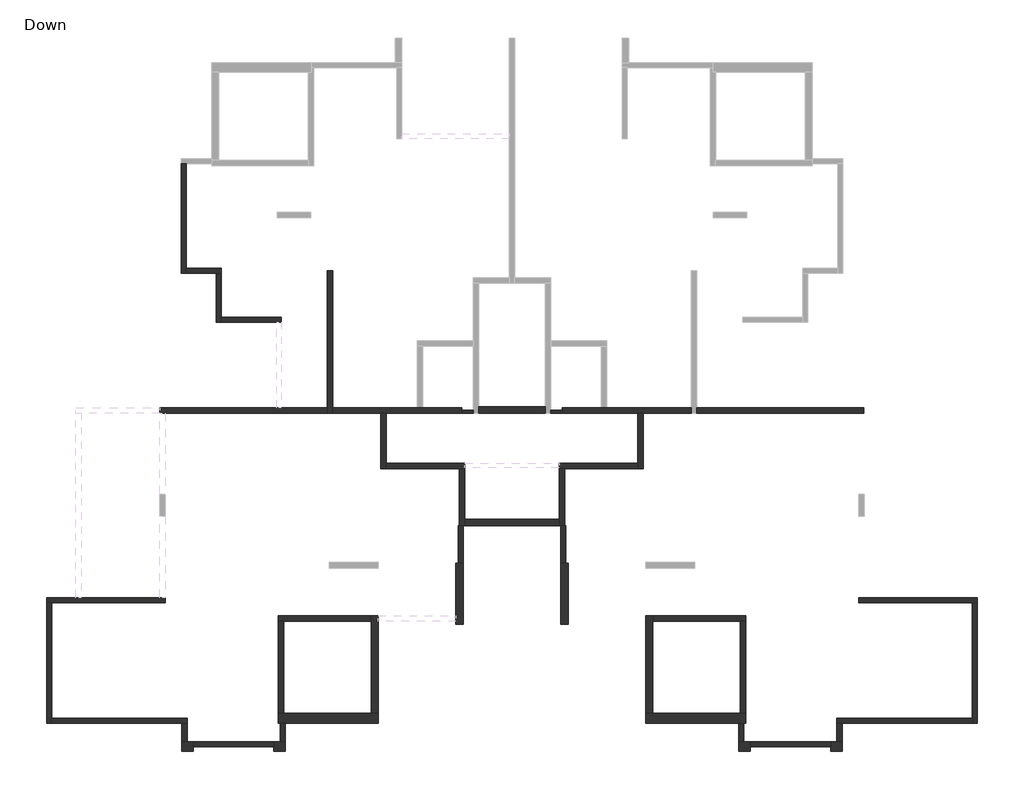
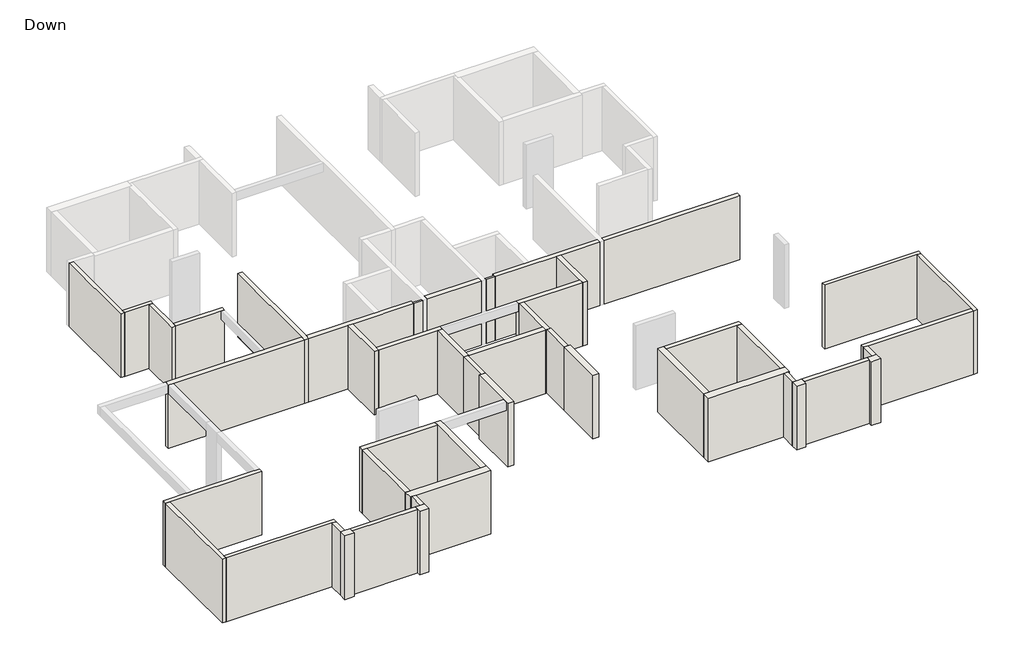
# One storey, part 1 of 2: 47 walls.
"""IFC4 building model written with IfcOpenShell, lengths in millimetres."""

import ifcopenshell
import ifcopenshell.guid

model = None  # the IFC model being written
_history = None  # IfcOwnerHistory: only IFC2X3 demands one
_inside = {}  # id of a spatial element -> (the spatial element, [elements in it])
_under = {}  # id of a project, library or spatial element -> (it, [spatial elements below it])
_declared = {}  # id of a project -> (the project, [libraries it declares])
_typed = {}  # id of a type object -> (the type object, [elements of that type])
_made_of = {}  # id of a material, layer set ... -> (it, [elements and type objects made of it])


def new_model(schema):
    """Start an empty IFC model of exactly this schema.

    Asked for "IFC4X3", IfcOpenShell would pick the latest addendum, in which some entities
    have other attributes; the version numbers below select the first issue.
    IFC2X3 requires an IfcOwnerHistory on every rooted entity: one is made here for all.
    """
    global model, _history
    if schema == "IFC4X3":
        model = ifcopenshell.file(schema_version=(4, 3, 0, 0))
    else:
        model = ifcopenshell.file(schema=schema)
    _inside.clear()
    _under.clear()
    _declared.clear()
    _typed.clear()
    _made_of.clear()
    _history = None
    if model.schema == "IFC2X3":
        org = make("IfcOrganization", Name="unknown")
        user = make(
            "IfcPersonAndOrganization",
            ThePerson=make("IfcPerson", FamilyName="unknown"),
            TheOrganization=org,
        )
        app = make(
            "IfcApplication",
            ApplicationDeveloper=org,
            Version="unknown",
            ApplicationFullName="unknown",
            ApplicationIdentifier="unknown",
        )
        _history = make(
            "IfcOwnerHistory",
            OwningUser=user,
            OwningApplication=app,
            ChangeAction="ADDED",
            CreationDate=0,
        )
    return model


def make(cls, **values):
    """One entity of the class cls with the attributes given. An attribute that is None is left unset."""
    return model.create_entity(
        cls, **{name: value for name, value in values.items() if value is not None}
    )


def rooted(cls, **values):
    """An entity with a GlobalId (a new one), such as an element, a storey or a relation."""
    return make(cls, GlobalId=ifcopenshell.guid.new(), OwnerHistory=_history, **values)


def si_unit(unit_type, name, prefix=None):
    """IfcSIUnit, for example si_unit("LENGTHUNIT", "METRE", prefix="MILLI")."""
    return make("IfcSIUnit", UnitType=unit_type, Prefix=prefix, Name=name)


def assignment(units):
    """IfcUnitAssignment: the units of a project."""
    return None if units is None else make("IfcUnitAssignment", Units=units)


def point(xyz):
    """IfcCartesianPoint."""
    return None if xyz is None else make("IfcCartesianPoint", Coordinates=xyz)


def direction(xyz):
    """IfcDirection."""
    return None if xyz is None else make("IfcDirection", DirectionRatios=xyz)


def frame(location, z_axis=None, x_axis=None):
    """IfcAxis2Placement3D, a coordinate frame: its origin and axes. An axis left out is left unset."""
    return make(
        "IfcAxis2Placement3D",
        Location=point(location),
        Axis=direction(z_axis),
        RefDirection=direction(x_axis),
    )


def origin():
    """The frame at (0, 0, 0) with its axes left unset."""
    return frame((0.0, 0.0, 0.0))


def origin_with_axes():
    """The frame at (0, 0, 0) with the z axis (0, 0, 1) and the x axis (1, 0, 0) written out."""
    return frame((0.0, 0.0, 0.0), z_axis=(0.0, 0.0, 1.0), x_axis=(1.0, 0.0, 0.0))


def place(relative_to, where):
    """IfcLocalPlacement: puts the frame where relative to a parent placement (None: the world)."""
    return make(
        "IfcLocalPlacement", PlacementRelTo=relative_to, RelativePlacement=where
    )


def context(
    kind, dimensions, precision=None, world=None, true_north=None, identifier=None
):
    """IfcGeometricRepresentationContext, for example the 3D "Model" context."""
    return make(
        "IfcGeometricRepresentationContext",
        ContextIdentifier=identifier,
        ContextType=kind,
        CoordinateSpaceDimension=dimensions,
        Precision=precision,
        WorldCoordinateSystem=world,
        TrueNorth=true_north,
    )


def project(units=None, contexts=None):
    """IfcProject with its units and contexts."""
    return rooted(
        "IfcProject",
        Name="project",
        RepresentationContexts=contexts,
        UnitsInContext=assignment(units),
    )


def spatial(cls, under=None, at=None, **own):
    """A site, building, storey or space (cls), placed at a placement, below another one or the project."""
    s = rooted(cls, ObjectPlacement=at, **own)
    if under is not None:
        _under.setdefault(under.id(), (under, []))[1].append(s)
    return s


def polyline(points):
    """IfcPolyline through the points."""
    return make("IfcPolyline", Points=[point(p) for p in points])


def outline(outer, holes=None, kind="AREA"):
    """IfcArbitraryClosedProfileDef: a profile drawn as a closed curve; with holes, ...WithVoids."""
    if holes is None:
        return make("IfcArbitraryClosedProfileDef", ProfileType=kind, OuterCurve=outer)
    return make(
        "IfcArbitraryProfileDefWithVoids",
        ProfileType=kind,
        OuterCurve=outer,
        InnerCurves=holes,
    )


def extrude(swept, where, along, depth):
    """IfcExtrudedAreaSolid: the profile swept, set in the frame where, extruded along a direction by depth."""
    return make(
        "IfcExtrudedAreaSolid",
        SweptArea=swept,
        Position=where,
        ExtrudedDirection=direction(along),
        Depth=depth,
    )


def faces_of(points, faces, orient=None, outer=None):
    """IfcFace entities. A face is a list of loops; a loop is a list of indices into points, from 0.

    orient and outer hold one flag for each loop. By default every Orientation is true, the
    first loop of a face is its IfcFaceOuterBound and the others are IfcFaceBound.
    """
    made = []
    for i, loops in enumerate(faces):
        bounds = []
        for j, loop in enumerate(loops):
            is_outer = j == 0 if outer is None else outer[i][j]
            bounds.append(
                make(
                    "IfcFaceOuterBound" if is_outer else "IfcFaceBound",
                    Bound=make("IfcPolyLoop", Polygon=[points[k] for k in loop]),
                    Orientation=True if orient is None else orient[i][j],
                )
            )
        made.append(make("IfcFace", Bounds=bounds))
    return made


def faceted_brep(points, faces, orient=None, outer=None, voids=None):
    """IfcFacetedBrep: a solid bounded by flat faces; with voids (closed shells), ...WithVoids."""
    shared = [point(p) for p in points]
    hull = make("IfcClosedShell", CfsFaces=faces_of(shared, faces, orient, outer))
    if voids is None:
        return make("IfcFacetedBrep", Outer=hull)
    return make(
        "IfcFacetedBrepWithVoids",
        Outer=hull,
        Voids=[
            make(cls, CfsFaces=faces_of(shared, fs, o, b)) for cls, fs, o, b in voids
        ],
    )


def shape(context_of_items, identifier, shape_type, items):
    """IfcShapeRepresentation: the items that make up one representation, for example the "Body"."""
    return make(
        "IfcShapeRepresentation",
        ContextOfItems=context_of_items,
        RepresentationIdentifier=identifier,
        RepresentationType=shape_type,
        Items=items,
    )


def made_of(thing, what):
    """Note that an element or type object is made of a material, layer set ...; save() writes the relation."""
    if what is not None:
        _made_of.setdefault(what.id(), (what, []))[1].append(thing)
    return thing


def element(
    cls,
    number,
    at=None,
    inside=None,
    cuts=None,
    type_object=None,
    material=None,
    context=None,
    identifier="Body",
    shape_type=None,
    held_by="IfcProductDefinitionShape",
    body=None,
    shapes=None,
    **own,
):
    """One element of the class cls, such as IfcWall. Its Tag is "e" and its number.

    at: its placement. inside: the storey or other place that contains it. cuts: it is an
    opening in that element (IfcRelVoidsElement). A single representation is given by context,
    identifier, shape_type and body (its items); several are given by shapes. held_by: the class
    of the entity that holds the representations. save() writes the other relations.
    """
    e = rooted(cls, Tag="e%d" % number, ObjectPlacement=at, **own)
    if body is not None:
        shapes = [shape(context, identifier, shape_type, body)]
    if shapes is not None:
        e.Representation = make(held_by, Representations=shapes)
    if inside is not None:
        _inside.setdefault(inside.id(), (inside, []))[1].append(e)
    if cuts is not None:
        rooted(
            "IfcRelVoidsElement", RelatingBuildingElement=cuts, RelatedOpeningElement=e
        )
    if type_object is not None:
        _typed.setdefault(type_object.id(), (type_object, []))[1].append(e)
    return made_of(e, material)


def aggregate(whole, parts):
    """IfcRelAggregates: a whole, such as a stair, and the parts it consists of."""
    return rooted("IfcRelAggregates", RelatingObject=whole, RelatedObjects=parts)


def save(model, path):
    """Write the relations noted so far, then the file.

    IfcRelAggregates (storeys below a building ...), IfcRelContainedInSpatialStructure (elements
    in a storey), IfcRelDefinesByType, IfcRelAssociatesMaterial and IfcRelDeclares: one each for
    every whole, place, type object, material and project.
    """
    for whole, parts in _under.values():
        aggregate(whole, parts)
    for where, things in _inside.values():
        rooted(
            "IfcRelContainedInSpatialStructure",
            RelatedElements=things,
            RelatingStructure=where,
        )
    for kind, things in _typed.values():
        rooted("IfcRelDefinesByType", RelatedObjects=things, RelatingType=kind)
    for what, things in _made_of.values():
        rooted("IfcRelAssociatesMaterial", RelatedObjects=things, RelatingMaterial=what)
    for by, libraries in _declared.values():
        rooted("IfcRelDeclares", RelatingContext=by, RelatedDefinitions=libraries)
    model.write(path)


model = new_model("IFC4")

# Units and contexts
model_context = context("Model", 3, world=origin())
ifc_project = project(units=[si_unit("LENGTHUNIT", "METRE", prefix="MILLI")], contexts=[model_context])

# Site, building, storey
site = spatial("IfcSite", under=ifc_project)
building = spatial("IfcBuilding", under=site)
storey = spatial("IfcBuildingStorey", under=building, Name="Down", Elevation=0.0)

# Walls
placement = place(None, origin())
element("IfcWall", 1, ObjectType="10", at=placement, inside=storey, context=model_context, shape_type="SweptSolid", body=[
    extrude(outline(polyline([(-572.4693797, -146.3653565), (-977.1774089, -146.3653565), (-977.1774089, -46.3653565), (-572.4693797, -46.3653565), (-572.4693797, -146.3653565)])), origin_with_axes(), (0.0, 0.0, 1.0), 2970.0),
])
element("IfcWall", 2, ObjectType="10", at=placement, inside=storey, context=model_context, shape_type="SweptSolid", body=[
    extrude(outline(polyline([(2217.5306203, -46.3653565), (2622.2386495, -46.3653565), (2622.2386495, -146.3653565), (2217.5306203, -146.3653565), (2217.5306203, -46.3653565)])), origin_with_axes(), (0.0, 0.0, 1.0), 2970.0),
])
element("IfcWall", 3, ObjectType="18", at=placement, inside=storey, context=model_context, shape_type="Brep", body=[
    faceted_brep([(-11023.126314, 8775.4959573, 0.0), (-11023.126314, 4855.4959573, 0.0), (-11023.126314, 4855.4959573, 2970.0), (-11023.126314, 8775.4959573, 2970.0), (-10843.126314, 8775.4959573, 0.0), (-10843.126314, 8775.4959573, 2760.0), (-10843.126314, 8775.4959573, 2970.0), (-10843.126314, 5035.4959573, 2970.0), (-10843.126314, 4855.4959573, 2970.0), (-10843.126314, 4855.4959573, 0.0), (-10843.126314, 5035.4959573, 0.0)], [[[0, 1, 2, 3]], [[4, 5, 6, 7, 8, 9, 10]], [[1, 0, 4, 10, 9]], [[3, 2, 8, 7, 6]], [[0, 3, 6, 5, 4]], [[2, 1, 9, 8]]]),
])
element("IfcWall", 4, ObjectType="18", at=placement, inside=storey, context=model_context, shape_type="Brep", body=[
    faceted_brep([(-10843.126314, 4855.4959573, 0.0), (-9775.6240301, 4855.4959573, 0.0), (-9595.6240301, 4855.4959573, 0.0), (-9595.6240301, 4855.4959573, 2970.0), (-9775.6240301, 4855.4959573, 2970.0), (-10843.126314, 4855.4959573, 2970.0), (-10843.126314, 5035.4959573, 0.0), (-10843.126314, 5035.4959573, 2760.0), (-10843.126314, 5035.4959573, 2970.0), (-9595.6240301, 5035.4959573, 2970.0), (-9595.6240301, 5035.4959573, 2760.0), (-9595.6240301, 5035.4959573, 0.0)], [[[0, 1, 2, 3, 4, 5]], [[6, 7, 8, 9, 10, 11]], [[2, 1, 0, 6, 11]], [[5, 4, 3, 9, 8]], [[0, 5, 8, 7, 6]], [[3, 2, 11, 10, 9]]]),
])
element("IfcWall", 5, ObjectType="18", at=placement, inside=storey, context=model_context, shape_type="Brep", body=[
    faceted_brep([(-9775.6240301, 4855.4959573, 0.0), (-9775.6240301, 3105.4959573, 0.0), (-9775.6240301, 3105.4959573, 2970.0), (-9775.6240301, 4855.4959573, 2970.0), (-9595.6240301, 4855.4959573, 0.0), (-9595.6240301, 4855.4959573, 2970.0), (-9595.6240301, 3285.4959573, 2970.0), (-9595.6240301, 3105.4959573, 2970.0), (-9595.6240301, 3105.4959573, 0.0), (-9595.6240301, 3285.4959573, 0.0)], [[[0, 1, 2, 3]], [[4, 5, 6, 7, 8, 9]], [[1, 0, 4, 9, 8]], [[3, 2, 7, 6, 5]], [[0, 3, 5, 4]], [[2, 1, 8, 7]]]),
])
element("IfcWall", 6, ObjectType="18", at=placement, inside=storey, context=model_context, shape_type="Brep", body=[
    faceted_brep([(-9595.6240301, 3105.4959573, 0.0), (-7445.6240301, 3105.4959573, 0.0), (-7445.6240301, 3105.4959573, 2760.0), (-7445.6240301, 3105.4959573, 2970.0), (-7447.2504016, 3105.4959573, 2970.0), (-9595.6240301, 3105.4959573, 2970.0), (-9595.6240301, 3285.4959573, 0.0), (-9595.6240301, 3285.4959573, 2760.0), (-9595.6240301, 3285.4959573, 2970.0), (-7445.6240301, 3285.4959573, 2970.0), (-7445.6240301, 3285.4959573, 2760.0), (-7445.6240301, 3285.4959573, 0.0)], [[[0, 1, 2, 3, 4, 5]], [[6, 7, 8, 9, 10, 11]], [[1, 0, 6, 11]], [[3, 2, 1, 11, 10, 9]], [[5, 4, 3, 9, 8]], [[0, 5, 8, 7, 6]]]),
])
element("IfcWall", 7, ObjectType="18", at=placement, inside=storey, context=model_context, shape_type="Brep", body=[
    faceted_brep([(-11593.7230475, -6750.8420555, 0.0), (-15843.7230475, -6750.8420555, 0.0), (-15843.7230475, -6750.8420555, 2970.0), (-14597.7613505, -6750.8420555, 2970.0), (-11795.1336133, -6750.8420555, 2970.0), (-11595.1336133, -6750.8420555, 2970.0), (-11593.7230475, -6750.8420555, 2970.0), (-11593.7230475, -6750.8420555, 2760.0), (-11593.7230475, -6930.8420555, 0.0), (-11593.7230475, -6930.8420555, 2760.0), (-11593.7230475, -6930.8420555, 2970.0), (-15663.7230475, -6930.8420555, 2970.0), (-15843.7230475, -6930.8420555, 2970.0), (-15843.7230475, -6930.8420555, 0.0), (-15663.7230475, -6930.8420555, 0.0)], [[[0, 1, 2, 3, 4, 5, 6, 7]], [[8, 9, 10, 11, 12, 13, 14]], [[1, 0, 8, 14, 13]], [[6, 5, 4, 3, 2, 12, 11, 10]], [[0, 7, 6, 10, 9, 8]], [[2, 1, 13, 12]]]),
])
element("IfcWall", 8, ObjectType="18", at=placement, inside=storey, context=model_context, shape_type="Brep", body=[
    faceted_brep([(-15843.7230475, -6930.8420555, 0.0), (-15843.7230475, -11250.8420555, 0.0), (-15843.7230475, -11250.8420555, 2970.0), (-15843.7230475, -6930.8420555, 2970.0), (-15663.7230475, -6930.8420555, 0.0), (-15663.7230475, -6930.8420555, 2760.0), (-15663.7230475, -6930.8420555, 2970.0), (-15663.7230475, -11070.8420555, 2970.0), (-15663.7230475, -11250.8420555, 2970.0), (-15663.7230475, -11250.8420555, 0.0), (-15663.7230475, -11070.8420555, 0.0)], [[[0, 1, 2, 3]], [[4, 5, 6, 7, 8, 9, 10]], [[1, 0, 4, 10, 9]], [[3, 2, 8, 7, 6]], [[0, 3, 6, 5, 4]], [[2, 1, 9, 8]]]),
])
element("IfcWall", 9, ObjectType="18", at=placement, inside=storey, context=model_context, shape_type="Brep", body=[
    faceted_brep([(-15663.7230475, -11250.8420555, 0.0), (-10993.7230475, -11250.8420555, 0.0), (-10813.7230475, -11250.8420555, 0.0), (-10813.7230475, -11250.8420555, 2970.0), (-10993.7230475, -11250.8420555, 2970.0), (-15663.7230475, -11250.8420555, 2970.0), (-15663.7230475, -11070.8420555, 0.0), (-15663.7230475, -11070.8420555, 2760.0), (-15663.7230475, -11070.8420555, 2970.0), (-10813.7230475, -11070.8420555, 2970.0), (-10813.7230475, -11070.8420555, 2760.0), (-10813.7230475, -11070.8420555, 0.0)], [[[0, 1, 2, 3, 4, 5]], [[6, 7, 8, 9, 10, 11]], [[2, 1, 0, 6, 11]], [[5, 4, 3, 9, 8]], [[0, 5, 8, 7, 6]], [[3, 2, 11, 10, 9]]]),
])
element("IfcWall", 10, ObjectType="18", at=placement, inside=storey, context=model_context, shape_type="Brep", body=[
    faceted_brep([(-10993.7230475, -11250.8420555, 0.0), (-10993.7230475, -11915.8420555, 0.0), (-10993.7230475, -11915.8420555, 2970.0), (-10993.7230475, -11250.8420555, 2970.0), (-10813.7230475, -11250.8420555, 0.0), (-10813.7230475, -11250.8420555, 2970.0), (-10813.7230475, -11915.8420555, 2970.0), (-10813.7230475, -11915.8420555, 2760.0), (-10813.7230475, -11915.8420555, 0.0)], [[[0, 1, 2, 3]], [[4, 5, 6, 7, 8]], [[1, 0, 4, 8]], [[3, 2, 6, 5]], [[0, 3, 5, 4]], [[2, 1, 8, 7, 6]]]),
])
element("IfcWall", 11, ObjectType="18", at=placement, inside=storey, context=model_context, shape_type="SweptSolid", body=[
    extrude(outline(polyline([(-7703.7230475, -12095.8420555), (-10588.7230475, -12095.8420555), (-10588.7230475, -11915.8420555), (-7703.7230475, -11915.8420555), (-7703.7230475, -12095.8420555)])), origin_with_axes(), (0.0, 0.0, 1.0), 2970.0),
])
element("IfcWall", 12, ObjectType="18", at=placement, inside=storey, context=model_context, shape_type="Brep", body=[
    faceted_brep([(-7293.7230475, -11915.8420555, 0.0), (-7293.7230475, -11245.8420555, 0.0), (-7293.7230475, -11245.8420555, 2970.0), (-7293.7230475, -11915.8420555, 2970.0), (-7473.7230475, -11915.8420555, 0.0), (-7473.7230475, -11915.8420555, 2760.0), (-7473.7230475, -11915.8420555, 2970.0), (-7473.7230475, -11245.8420555, 2970.0), (-7473.7230475, -11245.8420555, 2760.0), (-7473.7230475, -11245.8420555, 0.0)], [[[0, 1, 2, 3]], [[4, 5, 6, 7, 8, 9]], [[1, 0, 4, 9]], [[3, 2, 7, 6]], [[0, 3, 6, 5, 4]], [[2, 1, 9, 8, 7]]]),
])
element("IfcWall", 13, ObjectType="18", at=placement, inside=storey, context=model_context, shape_type="Brep", body=[
    faceted_brep([(-1099.5073169, -4176.3653565, 0.0), (-1099.5073169, -5521.3653565, 0.0), (-1099.5073169, -5521.3653565, 2760.0), (-1099.5073169, -5521.3653565, 2970.0), (-1099.5073169, -4176.3653565, 2970.0), (-1099.5073169, -4176.3653565, 2760.0), (-919.5073169, -4176.3653565, 0.0), (-919.5073169, -4176.3653565, 2970.0), (-919.5073169, -5521.3653565, 2970.0), (-919.5073169, -5521.3653565, 0.0), (-1074.5073169, -4176.3653565, 0.0), (-1074.5073169, -4176.3653565, 2970.0)], [[[0, 1, 2, 3, 4, 5]], [[6, 7, 8, 9]], [[1, 0, 10, 6, 9]], [[3, 2, 1, 9, 8]], [[4, 3, 8, 7, 11]], [[0, 5, 4, 11, 7, 6, 10]]]),
])
element("IfcWall", 14, ObjectType="18", at=placement, inside=storey, context=model_context, shape_type="Brep", body=[
    faceted_brep([(13238.7842881, -6930.8420555, 0.0), (17308.7842881, -6930.8420555, 0.0), (17488.7842881, -6930.8420555, 0.0), (17488.7842881, -6930.8420555, 2970.0), (17308.7842881, -6930.8420555, 2970.0), (13238.7842881, -6930.8420555, 2970.0), (13238.7842881, -6930.8420555, 2760.0), (13238.7842881, -6750.8420555, 0.0), (13238.7842881, -6750.8420555, 2760.0), (13238.7842881, -6750.8420555, 2970.0), (13240.1948538, -6750.8420555, 2970.0), (13440.1948538, -6750.8420555, 2970.0), (16242.8225911, -6750.8420555, 2970.0), (17488.7842881, -6750.8420555, 2970.0), (17488.7842881, -6750.8420555, 0.0)], [[[0, 1, 2, 3, 4, 5, 6]], [[7, 8, 9, 10, 11, 12, 13, 14]], [[2, 1, 0, 7, 14]], [[5, 4, 3, 13, 12, 11, 10, 9]], [[0, 6, 5, 9, 8, 7]], [[3, 2, 14, 13]]]),
])
element("IfcWall", 15, ObjectType="18", at=placement, inside=storey, context=model_context, shape_type="Brep", body=[
    faceted_brep([(17308.7842881, -6930.8420555, 0.0), (17308.7842881, -11070.8420555, 0.0), (17308.7842881, -11250.8420555, 0.0), (17308.7842881, -11250.8420555, 2970.0), (17308.7842881, -11070.8420555, 2970.0), (17308.7842881, -6930.8420555, 2970.0), (17308.7842881, -6930.8420555, 2760.0), (17488.7842881, -6930.8420555, 0.0), (17488.7842881, -6930.8420555, 2970.0), (17488.7842881, -11250.8420555, 2970.0), (17488.7842881, -11250.8420555, 0.0)], [[[0, 1, 2, 3, 4, 5, 6]], [[7, 8, 9, 10]], [[2, 1, 0, 7, 10]], [[5, 4, 3, 9, 8]], [[0, 6, 5, 8, 7]], [[3, 2, 10, 9]]]),
])
element("IfcWall", 16, ObjectType="18", at=placement, inside=storey, context=model_context, shape_type="Brep", body=[
    faceted_brep([(17308.7842881, -11070.8420555, 0.0), (12458.7842881, -11070.8420555, 0.0), (12458.7842881, -11070.8420555, 2760.0), (12458.7842881, -11070.8420555, 2970.0), (17308.7842881, -11070.8420555, 2970.0), (17308.7842881, -11070.8420555, 2760.0), (17308.7842881, -11250.8420555, 0.0), (17308.7842881, -11250.8420555, 2970.0), (12638.7842881, -11250.8420555, 2970.0), (12458.7842881, -11250.8420555, 2970.0), (12458.7842881, -11250.8420555, 0.0), (12638.7842881, -11250.8420555, 0.0)], [[[0, 1, 2, 3, 4, 5]], [[6, 7, 8, 9, 10, 11]], [[1, 0, 6, 11, 10]], [[4, 3, 9, 8, 7]], [[0, 5, 4, 7, 6]], [[3, 2, 1, 10, 9]]]),
])
element("IfcWall", 17, ObjectType="18", at=placement, inside=storey, context=model_context, shape_type="Brep", body=[
    faceted_brep([(12458.7842881, -11250.8420555, 0.0), (12458.7842881, -11915.8420555, 0.0), (12458.7842881, -11915.8420555, 2760.0), (12458.7842881, -11915.8420555, 2970.0), (12458.7842881, -11250.8420555, 2970.0), (12638.7842881, -11250.8420555, 0.0), (12638.7842881, -11250.8420555, 2970.0), (12638.7842881, -11915.8420555, 2970.0), (12638.7842881, -11915.8420555, 0.0)], [[[0, 1, 2, 3, 4]], [[5, 6, 7, 8]], [[1, 0, 5, 8]], [[4, 3, 7, 6]], [[0, 4, 6, 5]], [[3, 2, 1, 8, 7]]]),
])
element("IfcWall", 18, ObjectType="18", at=placement, inside=storey, context=model_context, shape_type="SweptSolid", body=[
    extrude(outline(polyline([(9348.7842881, -11915.8420555), (12233.7842881, -11915.8420555), (12233.7842881, -12095.8420555), (9348.7842881, -12095.8420555), (9348.7842881, -11915.8420555)])), origin_with_axes(), (0.0, 0.0, 1.0), 2970.0),
])
element("IfcWall", 19, ObjectType="18", at=placement, inside=storey, context=model_context, shape_type="Brep", body=[
    faceted_brep([(9118.7842881, -11915.8420555, 0.0), (9118.7842881, -11245.8420555, 0.0), (9118.7842881, -11245.8420555, 2760.0), (9118.7842881, -11245.8420555, 2970.0), (9118.7842881, -11915.8420555, 2970.0), (9118.7842881, -11915.8420555, 2760.0), (8938.7842881, -11915.8420555, 0.0), (8938.7842881, -11915.8420555, 2970.0), (8938.7842881, -11245.8420555, 2970.0), (8938.7842881, -11245.8420555, 0.0)], [[[0, 1, 2, 3, 4, 5]], [[6, 7, 8, 9]], [[1, 0, 6, 9]], [[4, 3, 8, 7]], [[0, 5, 4, 7, 6]], [[3, 2, 1, 9, 8]]]),
])
element("IfcWall", 20, ObjectType="18", at=placement, inside=storey, context=model_context, shape_type="Brep", body=[
    faceted_brep([(2564.5685574, -4176.3653565, 0.0), (2564.5685574, -5521.3653565, 0.0), (2564.5685574, -5521.3653565, 2970.0), (2564.5685574, -4176.3653565, 2970.0), (2744.5685574, -4176.3653565, 0.0), (2744.5685574, -4176.3653565, 2760.0), (2744.5685574, -4176.3653565, 2970.0), (2744.5685574, -5521.3653565, 2970.0), (2744.5685574, -5521.3653565, 2760.0), (2744.5685574, -5521.3653565, 0.0), (2719.5685574, -4176.3653565, 0.0), (2719.5685574, -4176.3653565, 2970.0)], [[[0, 1, 2, 3]], [[4, 5, 6, 7, 8, 9]], [[1, 0, 10, 4, 9]], [[2, 1, 9, 8, 7]], [[3, 2, 7, 6, 11]], [[0, 3, 11, 6, 5, 4, 10]]]),
])
element("IfcWall", 21, ObjectType="20", at=placement, inside=storey, context=model_context, shape_type="Brep", body=[
    faceted_brep([(-5797.1774089, 4958.6346435, 0.0), (-5797.1774089, 53.6346435, 0.0), (-5797.1774089, -146.3653565, 0.0), (-5797.1774089, -146.3653565, 2970.0), (-5797.1774089, 53.6346435, 2970.0), (-5797.1774089, 4958.6346435, 2970.0), (-5797.1774089, 4958.6346435, 2760.0), (-5597.1774089, 4958.6346435, 0.0), (-5597.1774089, 4958.6346435, 2760.0), (-5597.1774089, 4958.6346435, 2970.0), (-5597.1774089, 53.6346435, 2970.0), (-5597.1774089, -146.3653565, 2970.0), (-5597.1774089, -146.3653565, 0.0), (-5597.1774089, 53.6346435, 0.0)], [[[0, 1, 2, 3, 4, 5, 6]], [[7, 8, 9, 10, 11, 12, 13]], [[2, 1, 0, 7, 13, 12]], [[5, 4, 3, 11, 10, 9]], [[0, 6, 5, 9, 8, 7]], [[3, 2, 12, 11]]]),
])
element("IfcWall", 22, ObjectType="20", at=placement, inside=storey, context=model_context, shape_type="Brep", body=[
    faceted_brep([(-5797.1774089, 53.6346435, 0.0), (-11795.1336133, 53.6346435, 0.0), (-11795.1336133, 53.6346435, 2570.0), (-11795.1336133, 53.6346435, 2970.0), (-7447.2504016, 53.6346435, 2970.0), (-5797.1774089, 53.6346435, 2970.0), (-5797.1774089, 53.6346435, 2760.0), (-5797.1774089, -146.3653565, 0.0), (-5797.1774089, -146.3653565, 2970.0), (-11595.1336133, -146.3653565, 2970.0), (-11795.1336133, -146.3653565, 2970.0), (-11795.1336133, -146.3653565, 2570.0), (-11795.1336133, -146.3653565, 0.0)], [[[0, 1, 2, 3, 4, 5, 6]], [[7, 8, 9, 10, 11, 12]], [[1, 0, 7, 12]], [[3, 2, 1, 12, 11, 10]], [[5, 4, 3, 10, 9, 8]], [[0, 6, 5, 8, 7]]]),
])
element("IfcWall", 23, ObjectType="20", at=placement, inside=storey, context=model_context, shape_type="Brep", body=[
    faceted_brep([(-4223.7230475, -7395.8420555, 0.0), (-7543.7230475, -7395.8420555, 0.0), (-7543.7230475, -7395.8420555, 2760.0), (-7543.7230475, -7395.8420555, 2970.0), (-4223.7230475, -7395.8420555, 2970.0), (-4223.7230475, -7595.8420555, 0.0), (-4223.7230475, -7595.8420555, 2760.0), (-4223.7230475, -7595.8420555, 2970.0), (-7343.7230475, -7595.8420555, 2970.0), (-7543.7230475, -7595.8420555, 2970.0), (-7543.7230475, -7595.8420555, 0.0), (-7343.7230475, -7595.8420555, 0.0)], [[[0, 1, 2, 3, 4]], [[5, 6, 7, 8, 9, 10, 11]], [[1, 0, 5, 11, 10]], [[4, 3, 9, 8, 7]], [[0, 4, 7, 6, 5]], [[3, 2, 1, 10, 9]]]),
])
element("IfcWall", 24, ObjectType="20", at=placement, inside=storey, context=model_context, shape_type="Brep", body=[
    faceted_brep([(-7543.7230475, -7595.8420555, 0.0), (-7543.7230475, -10895.8420555, 0.0), (-7543.7230475, -10895.8420555, 2970.0), (-7543.7230475, -7595.8420555, 2970.0), (-7343.7230475, -7595.8420555, 0.0), (-7343.7230475, -7595.8420555, 2760.0), (-7343.7230475, -7595.8420555, 2970.0), (-7343.7230475, -10895.8420555, 2970.0), (-7343.7230475, -10895.8420555, 2760.0), (-7343.7230475, -10895.8420555, 0.0)], [[[0, 1, 2, 3]], [[4, 5, 6, 7, 8, 9]], [[1, 0, 4, 9]], [[3, 2, 7, 6]], [[0, 3, 6, 5, 4]], [[2, 1, 9, 8, 7]]]),
])
element("IfcWall", 25, ObjectType="20", at=placement, inside=storey, context=model_context, shape_type="Brep", body=[
    faceted_brep([(-5597.1774089, -146.3653565, 0.0), (-3874.5073169, -146.3653565, 0.0), (-3674.5073169, -146.3653565, 0.0), (-977.1774089, -146.3653565, 0.0), (-977.1774089, -146.3653565, 2970.0), (-3674.5073169, -146.3653565, 2970.0), (-3874.5073169, -146.3653565, 2970.0), (-5597.1774089, -146.3653565, 2970.0), (-5597.1774089, 53.6346435, 0.0), (-5597.1774089, 53.6346435, 2760.0), (-5597.1774089, 53.6346435, 2970.0), (-2572.4693797, 53.6346435, 2970.0), (-2372.4693797, 53.6346435, 2970.0), (-977.1774089, 53.6346435, 2970.0), (-977.1774089, 53.6346435, 0.0), (-2372.4693797, 53.6346435, 0.0), (-2572.4693797, 53.6346435, 0.0), (-977.1774089, -46.3653565, 0.0), (-977.1774089, -46.3653565, 2970.0)], [[[0, 1, 2, 3, 4, 5, 6, 7]], [[8, 9, 10, 11, 12, 13, 14, 15, 16]], [[3, 2, 1, 0, 8, 16, 15, 14, 17]], [[4, 3, 17, 14, 13, 18]], [[7, 6, 5, 4, 18, 13, 12, 11, 10]], [[0, 7, 10, 9, 8]]]),
])
element("IfcWall", 26, ObjectType="20", at=placement, inside=storey, context=model_context, shape_type="Brep", body=[
    faceted_brep([(-3874.5073169, -146.3653565, 0.0), (-3874.5073169, -2146.3653565, 0.0), (-3874.5073169, -2146.3653565, 2760.0), (-3874.5073169, -2146.3653565, 2970.0), (-3874.5073169, -146.3653565, 2970.0), (-3874.5073169, -146.3653565, 2760.0), (-3674.5073169, -146.3653565, 0.0), (-3674.5073169, -146.3653565, 2760.0), (-3674.5073169, -146.3653565, 2970.0), (-3674.5073169, -1946.3653565, 2970.0), (-3674.5073169, -2146.3653565, 2970.0), (-3674.5073169, -2146.3653565, 0.0), (-3674.5073169, -1946.3653565, 0.0)], [[[0, 1, 2, 3, 4, 5]], [[6, 7, 8, 9, 10, 11, 12]], [[1, 0, 6, 12, 11]], [[4, 3, 10, 9, 8]], [[0, 5, 4, 8, 7, 6]], [[3, 2, 1, 11, 10]]]),
])
element("IfcWall", 27, ObjectType="20", at=placement, inside=storey, context=model_context, shape_type="Brep", body=[
    faceted_brep([(-3674.5073169, -2146.3653565, 0.0), (-1074.5073169, -2146.3653565, 0.0), (-874.5073169, -2146.3653565, 0.0), (-874.5073169, -2146.3653565, 2970.0), (-1074.5073169, -2146.3653565, 2970.0), (-3674.5073169, -2146.3653565, 2970.0), (-3674.5073169, -1946.3653565, 0.0), (-3674.5073169, -1946.3653565, 2760.0), (-3674.5073169, -1946.3653565, 2970.0), (-874.5073169, -1946.3653565, 2970.0), (-874.5073169, -1946.3653565, 2570.0), (-874.5073169, -1946.3653565, 0.0), (-874.5073169, -2096.3653565, 2970.0)], [[[0, 1, 2, 3, 4, 5]], [[6, 7, 8, 9, 10, 11]], [[2, 1, 0, 6, 11]], [[5, 4, 3, 12, 9, 8]], [[0, 5, 8, 7, 6]], [[3, 2, 11, 10, 9, 12]]]),
])
element("IfcWall", 28, ObjectType="20", at=placement, inside=storey, context=model_context, shape_type="Brep", body=[
    faceted_brep([(-1074.5073169, -2146.3653565, 0.0), (-1074.5073169, -4176.3653565, 0.0), (-1074.5073169, -4176.3653565, 2760.0), (-1074.5073169, -4176.3653565, 2970.0), (-1074.5073169, -2146.3653565, 2970.0), (-1074.5073169, -2146.3653565, 2760.0), (-874.5073169, -2146.3653565, 0.0), (-874.5073169, -2146.3653565, 2970.0), (-874.5073169, -3946.3653565, 2970.0), (-874.5073169, -4176.3653565, 2970.0), (-874.5073169, -4176.3653565, 0.0), (-874.5073169, -3946.3653565, 0.0), (-919.5073169, -4176.3653565, 0.0), (-919.5073169, -4176.3653565, 2970.0)], [[[0, 1, 2, 3, 4, 5]], [[6, 7, 8, 9, 10, 11]], [[1, 0, 6, 11, 10, 12]], [[4, 3, 13, 9, 8, 7]], [[0, 5, 4, 7, 6]], [[3, 2, 1, 12, 10, 9, 13]]]),
])
element("IfcWall", 29, ObjectType="20", at=placement, inside=storey, context=model_context, shape_type="Brep", body=[
    faceted_brep([(7442.2386495, -146.3653565, 0.0), (13417.2386495, -146.3653565, 0.0), (13417.2386495, -146.3653565, 2570.0), (13417.2386495, -146.3653565, 2970.0), (13240.1948538, -146.3653565, 2970.0), (7442.2386495, -146.3653565, 2970.0), (7442.2386495, 53.6346435, 0.0), (7442.2386495, 53.6346435, 2760.0), (7442.2386495, 53.6346435, 2970.0), (9092.3116422, 53.6346435, 2970.0), (13417.2386495, 53.6346435, 2970.0), (13417.2386495, 53.6346435, 2570.0), (13417.2386495, 53.6346435, 0.0)], [[[0, 1, 2, 3, 4, 5]], [[6, 7, 8, 9, 10, 11, 12]], [[1, 0, 6, 12]], [[3, 2, 1, 12, 11, 10]], [[5, 4, 3, 10, 9, 8]], [[0, 5, 8, 7, 6]]]),
])
element("IfcWall", 30, ObjectType="20", at=placement, inside=storey, context=model_context, shape_type="Brep", body=[
    faceted_brep([(5868.7842881, -7595.8420555, 0.0), (8988.7842881, -7595.8420555, 0.0), (9188.7842881, -7595.8420555, 0.0), (9188.7842881, -7595.8420555, 2970.0), (8988.7842881, -7595.8420555, 2970.0), (5868.7842881, -7595.8420555, 2970.0), (5868.7842881, -7595.8420555, 2760.0), (5868.7842881, -7395.8420555, 0.0), (5868.7842881, -7395.8420555, 2970.0), (9188.7842881, -7395.8420555, 2970.0), (9188.7842881, -7395.8420555, 2760.0), (9188.7842881, -7395.8420555, 0.0)], [[[0, 1, 2, 3, 4, 5, 6]], [[7, 8, 9, 10, 11]], [[2, 1, 0, 7, 11]], [[5, 4, 3, 9, 8]], [[0, 6, 5, 8, 7]], [[3, 2, 11, 10, 9]]]),
])
element("IfcWall", 31, ObjectType="20", at=placement, inside=storey, context=model_context, shape_type="Brep", body=[
    faceted_brep([(8988.7842881, -7595.8420555, 0.0), (8988.7842881, -10895.8420555, 0.0), (8988.7842881, -10895.8420555, 2760.0), (8988.7842881, -10895.8420555, 2970.0), (8988.7842881, -7595.8420555, 2970.0), (8988.7842881, -7595.8420555, 2760.0), (9188.7842881, -7595.8420555, 0.0), (9188.7842881, -7595.8420555, 2970.0), (9188.7842881, -10895.8420555, 2970.0), (9188.7842881, -10895.8420555, 0.0)], [[[0, 1, 2, 3, 4, 5]], [[6, 7, 8, 9]], [[1, 0, 6, 9]], [[4, 3, 8, 7]], [[0, 5, 4, 7, 6]], [[3, 2, 1, 9, 8]]]),
])
element("IfcWall", 32, ObjectType="20", at=placement, inside=storey, context=model_context, shape_type="Brep", body=[
    faceted_brep([(7242.2386495, 53.6346435, 0.0), (4217.5306203, 53.6346435, 0.0), (4017.5306203, 53.6346435, 0.0), (2622.2386495, 53.6346435, 0.0), (2622.2386495, 53.6346435, 2970.0), (4017.5306203, 53.6346435, 2970.0), (4217.5306203, 53.6346435, 2970.0), (7242.2386495, 53.6346435, 2970.0), (7242.2386495, 53.6346435, 2760.0), (7242.2386495, -146.3653565, 0.0), (7242.2386495, -146.3653565, 2970.0), (5519.5685574, -146.3653565, 2970.0), (5319.5685574, -146.3653565, 2970.0), (2622.2386495, -146.3653565, 2970.0), (2622.2386495, -146.3653565, 0.0), (5319.5685574, -146.3653565, 0.0), (5519.5685574, -146.3653565, 0.0), (2622.2386495, -46.3653565, 0.0), (2622.2386495, -46.3653565, 2970.0)], [[[0, 1, 2, 3, 4, 5, 6, 7, 8]], [[9, 10, 11, 12, 13, 14, 15, 16]], [[3, 2, 1, 0, 9, 16, 15, 14, 17]], [[4, 3, 17, 14, 13, 18]], [[7, 6, 5, 4, 18, 13, 12, 11, 10]], [[0, 8, 7, 10, 9]]]),
])
element("IfcWall", 33, ObjectType="20", at=placement, inside=storey, context=model_context, shape_type="Brep", body=[
    faceted_brep([(5319.5685574, -146.3653565, 0.0), (5319.5685574, -1946.3653565, 0.0), (5319.5685574, -2146.3653565, 0.0), (5319.5685574, -2146.3653565, 2970.0), (5319.5685574, -1946.3653565, 2970.0), (5319.5685574, -146.3653565, 2970.0), (5319.5685574, -146.3653565, 2760.0), (5519.5685574, -146.3653565, 0.0), (5519.5685574, -146.3653565, 2760.0), (5519.5685574, -146.3653565, 2970.0), (5519.5685574, -2146.3653565, 2970.0), (5519.5685574, -2146.3653565, 2760.0), (5519.5685574, -2146.3653565, 0.0)], [[[0, 1, 2, 3, 4, 5, 6]], [[7, 8, 9, 10, 11, 12]], [[2, 1, 0, 7, 12]], [[5, 4, 3, 10, 9]], [[0, 6, 5, 9, 8, 7]], [[3, 2, 12, 11, 10]]]),
])
element("IfcWall", 34, ObjectType="20", at=placement, inside=storey, context=model_context, shape_type="Brep", body=[
    faceted_brep([(5319.5685574, -1946.3653565, 0.0), (2519.5685574, -1946.3653565, 0.0), (2519.5685574, -1946.3653565, 2570.0), (2519.5685574, -1946.3653565, 2970.0), (5319.5685574, -1946.3653565, 2970.0), (5319.5685574, -1946.3653565, 2760.0), (5319.5685574, -2146.3653565, 0.0), (5319.5685574, -2146.3653565, 2970.0), (2719.5685574, -2146.3653565, 2970.0), (2519.5685574, -2146.3653565, 2970.0), (2519.5685574, -2146.3653565, 0.0), (2719.5685574, -2146.3653565, 0.0), (2519.5685574, -2096.3653565, 2970.0)], [[[0, 1, 2, 3, 4, 5]], [[6, 7, 8, 9, 10, 11]], [[1, 0, 6, 11, 10]], [[4, 3, 12, 9, 8, 7]], [[0, 5, 4, 7, 6]], [[3, 2, 1, 10, 9, 12]]]),
])
element("IfcWall", 35, ObjectType="20", at=placement, inside=storey, context=model_context, shape_type="Brep", body=[
    faceted_brep([(2519.5685574, -2146.3653565, 0.0), (2519.5685574, -3946.3653565, 0.0), (2519.5685574, -4176.3653565, 0.0), (2519.5685574, -4176.3653565, 2970.0), (2519.5685574, -3946.3653565, 2970.0), (2519.5685574, -2146.3653565, 2970.0), (2719.5685574, -2146.3653565, 0.0), (2719.5685574, -2146.3653565, 2760.0), (2719.5685574, -2146.3653565, 2970.0), (2719.5685574, -4176.3653565, 2970.0), (2719.5685574, -4176.3653565, 2760.0), (2719.5685574, -4176.3653565, 0.0), (2564.5685574, -4176.3653565, 0.0), (2564.5685574, -4176.3653565, 2970.0)], [[[0, 1, 2, 3, 4, 5]], [[6, 7, 8, 9, 10, 11]], [[2, 1, 0, 6, 11, 12]], [[5, 4, 3, 13, 9, 8]], [[0, 5, 8, 7, 6]], [[3, 2, 12, 11, 10, 9, 13]]]),
])
element("IfcWall", 36, ObjectType="23", at=placement, inside=storey, context=model_context, shape_type="Brep", body=[
    faceted_brep([(-874.5073169, -4176.3653565, 0.0), (2519.5685574, -4176.3653565, 0.0), (2519.5685574, -4176.3653565, 2970.0), (-874.5073169, -4176.3653565, 2970.0), (-874.5073169, -3946.3653565, 0.0), (-874.5073169, -3946.3653565, 2760.0), (-874.5073169, -3946.3653565, 2970.0), (2519.5685574, -3946.3653565, 2970.0), (2519.5685574, -3946.3653565, 2760.0), (2519.5685574, -3946.3653565, 0.0)], [[[0, 1, 2, 3]], [[4, 5, 6, 7, 8, 9]], [[1, 0, 4, 9]], [[3, 2, 7, 6]], [[0, 3, 6, 5, 4]], [[2, 1, 9, 8, 7]]]),
])
element("IfcWall", 37, ObjectType="23", at=placement, inside=storey, context=model_context, shape_type="SweptSolid", body=[
    extrude(outline(polyline([(-372.4693797, 83.6346435), (2017.5306203, 83.6346435), (2017.5306203, -146.3653565), (-372.4693797, -146.3653565), (-372.4693797, 83.6346435)])), origin_with_axes(), (0.0, 0.0, 1.0), 2970.0),
])
element("IfcWall", 38, ObjectType="25", at=placement, inside=storey, context=model_context, shape_type="Brep", body=[
    faceted_brep([(-3973.7230475, -10895.8420555, 0.0), (-3973.7230475, -7395.8420555, 0.0), (-3973.7230475, -7395.8420555, 2970.0), (-3973.7230475, -10895.8420555, 2970.0), (-4223.7230475, -10895.8420555, 0.0), (-4223.7230475, -10895.8420555, 2760.0), (-4223.7230475, -10895.8420555, 2970.0), (-4223.7230475, -7595.8420555, 2970.0), (-4223.7230475, -7395.8420555, 2970.0), (-4223.7230475, -7395.8420555, 0.0), (-4223.7230475, -7595.8420555, 0.0)], [[[0, 1, 2, 3]], [[4, 5, 6, 7, 8, 9, 10]], [[1, 0, 4, 10, 9]], [[3, 2, 8, 7, 6]], [[0, 3, 6, 5, 4]], [[2, 1, 9, 8]]]),
])
element("IfcWall", 39, ObjectType="25", at=placement, inside=storey, context=model_context, shape_type="Brep", body=[
    faceted_brep([(5868.7842881, -10895.8420555, 0.0), (5868.7842881, -7595.8420555, 0.0), (5868.7842881, -7395.8420555, 0.0), (5868.7842881, -7395.8420555, 2970.0), (5868.7842881, -7595.8420555, 2970.0), (5868.7842881, -10895.8420555, 2970.0), (5868.7842881, -10895.8420555, 2760.0), (5618.7842881, -10895.8420555, 0.0), (5618.7842881, -10895.8420555, 2970.0), (5618.7842881, -7395.8420555, 2970.0), (5618.7842881, -7395.8420555, 0.0)], [[[0, 1, 2, 3, 4, 5, 6]], [[7, 8, 9, 10]], [[2, 1, 0, 7, 10]], [[5, 4, 3, 9, 8]], [[0, 6, 5, 8, 7]], [[3, 2, 10, 9]]]),
])
element("IfcWall", 40, ObjectType="27", at=placement, inside=storey, context=model_context, shape_type="Brep", body=[
    faceted_brep([(-1189.5073169, -5521.3653565, 0.0), (-1189.5073169, -7701.3653565, 0.0), (-1189.5073169, -7701.3653565, 2970.0), (-1189.5073169, -7395.8420555, 2970.0), (-1189.5073169, -5521.3653565, 2970.0), (-1189.5073169, -5521.3653565, 2760.0), (-919.5073169, -5521.3653565, 0.0), (-919.5073169, -5521.3653565, 2970.0), (-919.5073169, -7701.3653565, 2970.0), (-919.5073169, -7701.3653565, 0.0), (-1099.5073169, -5521.3653565, 0.0), (-1099.5073169, -5521.3653565, 2970.0)], [[[0, 1, 2, 3, 4, 5]], [[6, 7, 8, 9]], [[1, 0, 10, 6, 9]], [[2, 1, 9, 8]], [[4, 3, 2, 8, 7, 11]], [[0, 5, 4, 11, 7, 6, 10]]]),
])
element("IfcWall", 41, ObjectType="27", at=placement, inside=storey, context=model_context, shape_type="Brep", body=[
    faceted_brep([(2564.5685574, -5521.3653565, 0.0), (2564.5685574, -7701.3653565, 0.0), (2564.5685574, -7701.3653565, 2970.0), (2564.5685574, -5521.3653565, 2970.0), (2834.5685574, -5521.3653565, 0.0), (2834.5685574, -5521.3653565, 2760.0), (2834.5685574, -5521.3653565, 2970.0), (2834.5685574, -7395.8420555, 2970.0), (2834.5685574, -7701.3653565, 2970.0), (2834.5685574, -7701.3653565, 0.0), (2744.5685574, -5521.3653565, 0.0), (2744.5685574, -5521.3653565, 2970.0)], [[[0, 1, 2, 3]], [[4, 5, 6, 7, 8, 9]], [[1, 0, 10, 4, 9]], [[2, 1, 9, 8]], [[3, 2, 8, 7, 6, 11]], [[0, 3, 11, 6, 5, 4, 10]]]),
])
element("IfcWall", 42, ObjectType="33", at=placement, inside=storey, context=model_context, shape_type="Brep", body=[
    faceted_brep([(-10993.7230475, -12245.8420555, 0.0), (-10588.7230475, -12245.8420555, 0.0), (-10588.7230475, -12245.8420555, 2970.0), (-10993.7230475, -12245.8420555, 2970.0), (-10993.7230475, -11915.8420555, 0.0), (-10993.7230475, -11915.8420555, 2970.0), (-10813.7230475, -11915.8420555, 2970.0), (-10588.7230475, -11915.8420555, 2970.0), (-10588.7230475, -11915.8420555, 0.0), (-10813.7230475, -11915.8420555, 0.0), (-10588.7230475, -12095.8420555, 0.0), (-10588.7230475, -12095.8420555, 2970.0)], [[[0, 1, 2, 3]], [[4, 5, 6, 7, 8, 9]], [[1, 0, 4, 9, 8, 10]], [[2, 1, 10, 8, 7, 11]], [[3, 2, 11, 7, 6, 5]], [[0, 3, 5, 4]]]),
])
element("IfcWall", 43, ObjectType="33", at=placement, inside=storey, context=model_context, shape_type="Brep", body=[
    faceted_brep([(-7293.7230475, -11915.8420555, 0.0), (-7473.7230475, -11915.8420555, 0.0), (-7703.7230475, -11915.8420555, 0.0), (-7703.7230475, -11915.8420555, 2970.0), (-7473.7230475, -11915.8420555, 2970.0), (-7293.7230475, -11915.8420555, 2970.0), (-7293.7230475, -12245.8420555, 0.0), (-7293.7230475, -12245.8420555, 2970.0), (-7703.7230475, -12245.8420555, 2970.0), (-7703.7230475, -12245.8420555, 0.0), (-7703.7230475, -12095.8420555, 0.0), (-7703.7230475, -12095.8420555, 2970.0)], [[[0, 1, 2, 3, 4, 5]], [[6, 7, 8, 9]], [[2, 1, 0, 6, 9, 10]], [[3, 2, 10, 9, 8, 11]], [[5, 4, 3, 11, 8, 7]], [[0, 5, 7, 6]]]),
])
element("IfcWall", 44, ObjectType="33", at=placement, inside=storey, context=model_context, shape_type="Brep", body=[
    faceted_brep([(12638.7842881, -11915.8420555, 0.0), (12458.7842881, -11915.8420555, 0.0), (12233.7842881, -11915.8420555, 0.0), (12233.7842881, -11915.8420555, 2970.0), (12458.7842881, -11915.8420555, 2970.0), (12638.7842881, -11915.8420555, 2970.0), (12638.7842881, -12245.8420555, 0.0), (12638.7842881, -12245.8420555, 2970.0), (12233.7842881, -12245.8420555, 2970.0), (12233.7842881, -12245.8420555, 0.0), (12233.7842881, -12095.8420555, 0.0), (12233.7842881, -12095.8420555, 2970.0)], [[[0, 1, 2, 3, 4, 5]], [[6, 7, 8, 9]], [[2, 1, 0, 6, 9, 10]], [[3, 2, 10, 9, 8, 11]], [[5, 4, 3, 11, 8, 7]], [[0, 5, 7, 6]]]),
])
element("IfcWall", 45, ObjectType="33", at=placement, inside=storey, context=model_context, shape_type="Brep", body=[
    faceted_brep([(8938.7842881, -12245.8420555, 0.0), (9348.7842881, -12245.8420555, 0.0), (9348.7842881, -12245.8420555, 2970.0), (8938.7842881, -12245.8420555, 2970.0), (8938.7842881, -11915.8420555, 0.0), (8938.7842881, -11915.8420555, 2970.0), (9118.7842881, -11915.8420555, 2970.0), (9348.7842881, -11915.8420555, 2970.0), (9348.7842881, -11915.8420555, 0.0), (9118.7842881, -11915.8420555, 0.0), (9348.7842881, -12095.8420555, 0.0), (9348.7842881, -12095.8420555, 2970.0)], [[[0, 1, 2, 3]], [[4, 5, 6, 7, 8, 9]], [[1, 0, 4, 9, 8, 10]], [[2, 1, 10, 8, 7, 11]], [[3, 2, 11, 7, 6, 5]], [[0, 3, 5, 4]]]),
])
element("IfcWall", 46, ObjectType="35", at=placement, inside=storey, context=model_context, shape_type="Brep", body=[
    faceted_brep([(-7543.7230475, -11245.8420555, 0.0), (-7473.7230475, -11245.8420555, 0.0), (-7293.7230475, -11245.8420555, 0.0), (-3973.7230475, -11245.8420555, 0.0), (-3973.7230475, -11245.8420555, 2970.0), (-7293.7230475, -11245.8420555, 2970.0), (-7473.7230475, -11245.8420555, 2970.0), (-7543.7230475, -11245.8420555, 2970.0), (-7543.7230475, -11245.8420555, 2760.0), (-7543.7230475, -10895.8420555, 0.0), (-7543.7230475, -10895.8420555, 2970.0), (-7343.7230475, -10895.8420555, 2970.0), (-4223.7230475, -10895.8420555, 2970.0), (-3973.7230475, -10895.8420555, 2970.0), (-3973.7230475, -10895.8420555, 0.0), (-4223.7230475, -10895.8420555, 0.0), (-7343.7230475, -10895.8420555, 0.0)], [[[0, 1, 2, 3, 4, 5, 6, 7, 8]], [[9, 10, 11, 12, 13, 14, 15, 16]], [[3, 2, 1, 0, 9, 16, 15, 14]], [[7, 6, 5, 4, 13, 12, 11, 10]], [[4, 3, 14, 13]], [[0, 8, 7, 10, 9]]]),
])
element("IfcWall", 47, ObjectType="35", at=placement, inside=storey, context=model_context, shape_type="Brep", body=[
    faceted_brep([(9188.7842881, -10895.8420555, 0.0), (8988.7842881, -10895.8420555, 0.0), (5868.7842881, -10895.8420555, 0.0), (5618.7842881, -10895.8420555, 0.0), (5618.7842881, -10895.8420555, 2970.0), (5868.7842881, -10895.8420555, 2970.0), (8988.7842881, -10895.8420555, 2970.0), (9188.7842881, -10895.8420555, 2970.0), (9188.7842881, -11245.8420555, 0.0), (9188.7842881, -11245.8420555, 2760.0), (9188.7842881, -11245.8420555, 2970.0), (9118.7842881, -11245.8420555, 2970.0), (8938.7842881, -11245.8420555, 2970.0), (5618.7842881, -11245.8420555, 2970.0), (5618.7842881, -11245.8420555, 0.0), (8938.7842881, -11245.8420555, 0.0), (9118.7842881, -11245.8420555, 0.0)], [[[0, 1, 2, 3, 4, 5, 6, 7]], [[8, 9, 10, 11, 12, 13, 14, 15, 16]], [[3, 2, 1, 0, 8, 16, 15, 14]], [[7, 6, 5, 4, 13, 12, 11, 10]], [[4, 3, 14, 13]], [[0, 7, 10, 9, 8]]]),
])

save(model, "model.ifc")

# Revit data of these elements
# Project information
#   Project Issue Date = "Issue Date"
#   Project Status = "Project Status"
#   Client Name = "לקוח"
#   Project Address = "Enter address here"
#   Project Name = "Project 012"
#   Project Number = "מספר פרויקט"
# Type "10"
#   Layers, outside or top first: 10 cm "Concrete" (function 1)
# Type "18"
#   Layers, outside or top first: 18 cm "Concrete" (function 1)
# Type "20"
#   Layers, outside or top first: 20 cm "Concrete" (function 1)
# Type "23"
#   Layers, outside or top first: 23 cm "Concrete" (function 1)
# Type "25"
#   Layers, outside or top first: 25 cm "Concrete" (function 1)
# Type "27"
#   Layers, outside or top first: 27 cm "Concrete" (function 1)
# Type "33"
#   Layers, outside or top first: 33 cm "Concrete" (function 1)
# Type "35"
#   Layers, outside or top first: 35 cm "Concrete" (function 1)
# Element 1 (IfcWall, "10")
#   Comments = ""
#   Mark = "W74"
#   SOFiSTiK_EdgeZones = "W74"
#   SOFiSTiK_AMG_Comments = "Too Narrow /"
#   Top Offset = 0 cm
#   Base Offset = 0 cm
#   wall height = 297 cm
#   SOFiSTiK_AMG_Scheduled = yes
#   SOFiSTiK_AMG_Adjusted = yes
#   Phase Created = New Construction
#   Base Constraint = Down
#   Top Constraint = Typical Floor
#   Materials on its faces: "Concrete"
# Element 2 (IfcWall, "10")
#   Comments = ""
#   Mark = "W75"
#   SOFiSTiK_EdgeZones = "W75"
#   SOFiSTiK_AMG_Comments = "Too Narrow /"
#   Top Offset = 0 cm
#   Base Offset = 0 cm
#   wall height = 297 cm
#   SOFiSTiK_AMG_Scheduled = yes
#   SOFiSTiK_AMG_Adjusted = yes
#   Phase Created = New Construction
#   Base Constraint = Down
#   Top Constraint = Typical Floor
#   Materials on its faces: "Concrete"
# Element 3 (IfcWall, "18")
#   Comments = ""
#   Mark = "W8"
#   SOFiSTiK_EdgeZones = "W8"
#   SOFiSTiK_AMG_Comments = ""
#   Top Offset = 0 cm
#   Base Offset = 0 cm
#   wall height = 297 cm
#   SOFiSTiK_AMG_Scheduled = yes
#   SOFiSTiK_AMG_Adjusted = yes
#   Phase Created = New Construction
#   Base Constraint = Down
#   Top Constraint = Typical Floor
#   Materials on its faces: "Concrete"
# Element 4 (IfcWall, "18")
#   Comments = ""
#   Mark = "W9"
#   SOFiSTiK_EdgeZones = "W9"
#   SOFiSTiK_AMG_Comments = ""
#   Top Offset = 0 cm
#   Base Offset = 0 cm
#   wall height = 297 cm
#   SOFiSTiK_AMG_Scheduled = yes
#   SOFiSTiK_AMG_Adjusted = yes
#   Phase Created = New Construction
#   Base Constraint = Down
#   Top Constraint = Typical Floor
#   Materials on its faces: "Concrete"
# Element 5 (IfcWall, "18")
#   Comments = ""
#   Mark = "W10"
#   SOFiSTiK_EdgeZones = "W10"
#   SOFiSTiK_AMG_Comments = ""
#   Top Offset = 0 cm
#   Base Offset = 0 cm
#   wall height = 297 cm
#   SOFiSTiK_AMG_Scheduled = yes
#   SOFiSTiK_AMG_Adjusted = yes
#   Phase Created = New Construction
#   Base Constraint = Down
#   Top Constraint = Typical Floor
#   Materials on its faces: "Concrete"
# Element 6 (IfcWall, "18")
#   Comments = ""
#   Mark = "W11"
#   SOFiSTiK_EdgeZones = "W11"
#   SOFiSTiK_AMG_Comments = ""
#   Top Offset = 0 cm
#   Base Offset = 0 cm
#   wall height = 297 cm
#   SOFiSTiK_AMG_Scheduled = yes
#   SOFiSTiK_AMG_Adjusted = yes
#   Phase Created = New Construction
#   Base Constraint = Down
#   Top Constraint = Typical Floor
#   Materials on its faces: "Concrete"
# Element 7 (IfcWall, "18")
#   Comments = ""
#   Mark = "W12"
#   SOFiSTiK_EdgeZones = "W12"
#   SOFiSTiK_AMG_Comments = ""
#   Top Offset = 0 cm
#   Base Offset = 0 cm
#   wall height = 297 cm
#   SOFiSTiK_AMG_Scheduled = yes
#   SOFiSTiK_AMG_Adjusted = yes
#   Phase Created = New Construction
#   Base Constraint = Down
#   Top Constraint = Typical Floor
#   Materials on its faces: "Concrete"
# Element 8 (IfcWall, "18")
#   Comments = ""
#   Mark = "W13"
#   SOFiSTiK_EdgeZones = "W13"
#   SOFiSTiK_AMG_Comments = ""
#   Top Offset = 0 cm
#   Base Offset = 0 cm
#   wall height = 297 cm
#   SOFiSTiK_AMG_Scheduled = yes
#   SOFiSTiK_AMG_Adjusted = yes
#   Phase Created = New Construction
#   Base Constraint = Down
#   Top Constraint = Typical Floor
#   Materials on its faces: "Concrete"
# Element 9 (IfcWall, "18")
#   Comments = ""
#   Mark = "W14"
#   SOFiSTiK_EdgeZones = "W14"
#   SOFiSTiK_AMG_Comments = ""
#   Top Offset = 0 cm
#   Base Offset = 0 cm
#   wall height = 297 cm
#   SOFiSTiK_AMG_Scheduled = yes
#   SOFiSTiK_AMG_Adjusted = yes
#   Phase Created = New Construction
#   Base Constraint = Down
#   Top Constraint = Typical Floor
#   Materials on its faces: "Concrete"
# Element 10 (IfcWall, "18")
#   Comments = ""
#   Mark = "W15"
#   SOFiSTiK_EdgeZones = "W15"
#   SOFiSTiK_AMG_Comments = ""
#   Top Offset = 0 cm
#   Base Offset = 0 cm
#   wall height = 297 cm
#   SOFiSTiK_AMG_Scheduled = yes
#   SOFiSTiK_AMG_Adjusted = yes
#   Phase Created = New Construction
#   Base Constraint = Down
#   Top Constraint = Typical Floor
#   Materials on its faces: "Concrete"
# Element 11 (IfcWall, "18")
#   Comments = ""
#   Mark = "W16"
#   SOFiSTiK_EdgeZones = "W16"
#   SOFiSTiK_AMG_Comments = ""
#   Top Offset = 0 cm
#   Base Offset = 0 cm
#   wall height = 297 cm
#   SOFiSTiK_AMG_Scheduled = yes
#   SOFiSTiK_AMG_Adjusted = yes
#   Phase Created = New Construction
#   Base Constraint = Down
#   Top Constraint = Typical Floor
#   Materials on its faces: "Concrete"
# Element 12 (IfcWall, "18")
#   Comments = ""
#   Mark = "W17"
#   SOFiSTiK_EdgeZones = "W17"
#   SOFiSTiK_AMG_Comments = ""
#   Top Offset = 0 cm
#   Base Offset = 0 cm
#   wall height = 297 cm
#   SOFiSTiK_AMG_Scheduled = yes
#   SOFiSTiK_AMG_Adjusted = yes
#   Phase Created = New Construction
#   Base Constraint = Down
#   Top Constraint = Typical Floor
#   Materials on its faces: "Concrete"
# Element 13 (IfcWall, "18")
#   Comments = ""
#   Mark = "W18"
#   SOFiSTiK_EdgeZones = "W18"
#   SOFiSTiK_AMG_Comments = ""
#   Top Offset = 0 cm
#   Base Offset = 0 cm
#   wall height = 297 cm
#   SOFiSTiK_AMG_Scheduled = yes
#   SOFiSTiK_AMG_Adjusted = yes
#   Phase Created = New Construction
#   Base Constraint = Down
#   Top Constraint = Typical Floor
#   Materials on its faces: "Concrete"
# Element 14 (IfcWall, "18")
#   Comments = ""
#   Mark = "W26"
#   SOFiSTiK_EdgeZones = "W26"
#   SOFiSTiK_AMG_Comments = ""
#   Top Offset = 0 cm
#   Base Offset = 0 cm
#   wall height = 297 cm
#   SOFiSTiK_AMG_Scheduled = yes
#   SOFiSTiK_AMG_Adjusted = yes
#   Phase Created = New Construction
#   Base Constraint = Down
#   Top Constraint = Typical Floor
#   Materials on its faces: "Concrete"
# Element 15 (IfcWall, "18")
#   Comments = ""
#   Mark = "W27"
#   SOFiSTiK_EdgeZones = "W27"
#   SOFiSTiK_AMG_Comments = ""
#   Top Offset = 0 cm
#   Base Offset = 0 cm
#   wall height = 297 cm
#   SOFiSTiK_AMG_Scheduled = yes
#   SOFiSTiK_AMG_Adjusted = yes
#   Phase Created = New Construction
#   Base Constraint = Down
#   Top Constraint = Typical Floor
#   Materials on its faces: "Concrete"
# Element 16 (IfcWall, "18")
#   Comments = ""
#   Mark = "W28"
#   SOFiSTiK_EdgeZones = "W28"
#   SOFiSTiK_AMG_Comments = ""
#   Top Offset = 0 cm
#   Base Offset = 0 cm
#   wall height = 297 cm
#   SOFiSTiK_AMG_Scheduled = yes
#   SOFiSTiK_AMG_Adjusted = yes
#   Phase Created = New Construction
#   Base Constraint = Down
#   Top Constraint = Typical Floor
#   Materials on its faces: "Concrete"
# Element 17 (IfcWall, "18")
#   Comments = ""
#   Mark = "W29"
#   SOFiSTiK_EdgeZones = "W29"
#   SOFiSTiK_AMG_Comments = ""
#   Top Offset = 0 cm
#   Base Offset = 0 cm
#   wall height = 297 cm
#   SOFiSTiK_AMG_Scheduled = yes
#   SOFiSTiK_AMG_Adjusted = yes
#   Phase Created = New Construction
#   Base Constraint = Down
#   Top Constraint = Typical Floor
#   Materials on its faces: "Concrete"
# Element 18 (IfcWall, "18")
#   Comments = ""
#   Mark = "W30"
#   SOFiSTiK_EdgeZones = "W30"
#   SOFiSTiK_AMG_Comments = ""
#   Top Offset = 0 cm
#   Base Offset = 0 cm
#   wall height = 297 cm
#   SOFiSTiK_AMG_Scheduled = yes
#   SOFiSTiK_AMG_Adjusted = yes
#   Phase Created = New Construction
#   Base Constraint = Down
#   Top Constraint = Typical Floor
#   Materials on its faces: "Concrete"
# Element 19 (IfcWall, "18")
#   Comments = ""
#   Mark = "W31"
#   SOFiSTiK_EdgeZones = "W31"
#   SOFiSTiK_AMG_Comments = ""
#   Top Offset = 0 cm
#   Base Offset = 0 cm
#   wall height = 297 cm
#   SOFiSTiK_AMG_Scheduled = yes
#   SOFiSTiK_AMG_Adjusted = yes
#   Phase Created = New Construction
#   Base Constraint = Down
#   Top Constraint = Typical Floor
#   Materials on its faces: "Concrete"
# Element 20 (IfcWall, "18")
#   Comments = ""
#   Mark = "W32"
#   SOFiSTiK_EdgeZones = "W32"
#   SOFiSTiK_AMG_Comments = ""
#   Top Offset = 0 cm
#   Base Offset = 0 cm
#   wall height = 297 cm
#   SOFiSTiK_AMG_Scheduled = yes
#   SOFiSTiK_AMG_Adjusted = yes
#   Phase Created = New Construction
#   Base Constraint = Down
#   Top Constraint = Typical Floor
#   Materials on its faces: "Concrete"
# Element 21 (IfcWall, "20")
#   Comments = ""
#   Mark = "W39"
#   SOFiSTiK_EdgeZones = "W39"
#   SOFiSTiK_AMG_Comments = ""
#   Top Offset = 0 cm
#   Base Offset = 0 cm
#   wall height = 297 cm
#   SOFiSTiK_AMG_Scheduled = yes
#   SOFiSTiK_AMG_Adjusted = yes
#   Phase Created = New Construction
#   Base Constraint = Down
#   Top Constraint = Typical Floor
#   Materials on its faces: "Concrete"
# Element 22 (IfcWall, "20")
#   Comments = ""
#   Mark = "W40"
#   SOFiSTiK_EdgeZones = "W40"
#   SOFiSTiK_AMG_Comments = ""
#   Top Offset = 0 cm
#   Base Offset = 0 cm
#   wall height = 297 cm
#   SOFiSTiK_AMG_Scheduled = yes
#   SOFiSTiK_AMG_Adjusted = yes
#   Phase Created = New Construction
#   Base Constraint = Down
#   Top Constraint = Typical Floor
#   Materials on its faces: "Concrete"
# Element 23 (IfcWall, "20")
#   Comments = ""
#   Mark = "W41"
#   SOFiSTiK_EdgeZones = "W41"
#   SOFiSTiK_AMG_Comments = ""
#   Top Offset = 0 cm
#   Base Offset = 0 cm
#   wall height = 297 cm
#   SOFiSTiK_AMG_Scheduled = yes
#   SOFiSTiK_AMG_Adjusted = yes
#   Phase Created = New Construction
#   Base Constraint = Down
#   Top Constraint = Typical Floor
#   Materials on its faces: "Concrete"
# Element 24 (IfcWall, "20")
#   Comments = ""
#   Mark = "W42"
